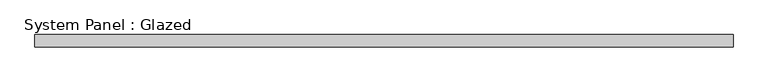
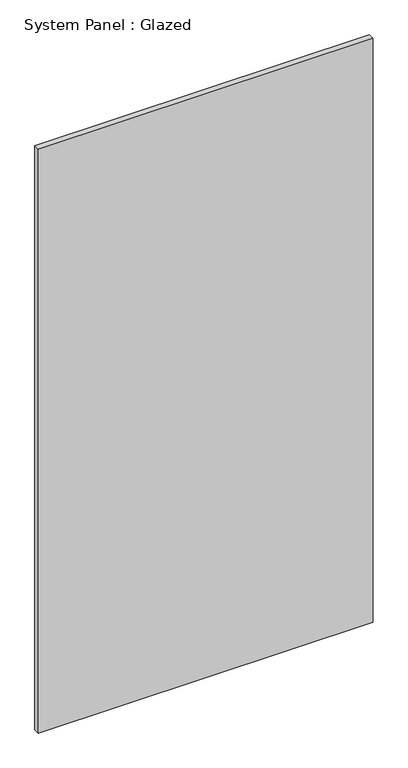
"""IFC4 building model written with IfcOpenShell, lengths in millimetres: plate geometry, System Panel : Glazed."""

import ifcopenshell
import ifcopenshell.guid

model = None  # the IFC model being written
_history = None  # IfcOwnerHistory: only IFC2X3 demands one
_inside = {}  # id of a spatial element -> (the spatial element, [elements in it])
_under = {}  # id of a project, library or spatial element -> (it, [spatial elements below it])
_declared = {}  # id of a project -> (the project, [libraries it declares])
_typed = {}  # id of a type object -> (the type object, [elements of that type])
_made_of = {}  # id of a material, layer set ... -> (it, [elements and type objects made of it])


def new_model(schema):
    """Start an empty IFC model of exactly this schema.

    Asked for "IFC4X3", IfcOpenShell would pick the latest addendum, in which some entities
    have other attributes; the version numbers below select the first issue.
    IFC2X3 requires an IfcOwnerHistory on every rooted entity: one is made here for all.
    """
    global model, _history
    if schema == "IFC4X3":
        model = ifcopenshell.file(schema_version=(4, 3, 0, 0))
    else:
        model = ifcopenshell.file(schema=schema)
    _inside.clear()
    _under.clear()
    _declared.clear()
    _typed.clear()
    _made_of.clear()
    _history = None
    if model.schema == "IFC2X3":
        org = make("IfcOrganization", Name="unknown")
        user = make(
            "IfcPersonAndOrganization",
            ThePerson=make("IfcPerson", FamilyName="unknown"),
            TheOrganization=org,
        )
        app = make(
            "IfcApplication",
            ApplicationDeveloper=org,
            Version="unknown",
            ApplicationFullName="unknown",
            ApplicationIdentifier="unknown",
        )
        _history = make(
            "IfcOwnerHistory",
            OwningUser=user,
            OwningApplication=app,
            ChangeAction="ADDED",
            CreationDate=0,
        )
    return model


def make(cls, **values):
    """One entity of the class cls with the attributes given. An attribute that is None is left unset."""
    return model.create_entity(
        cls, **{name: value for name, value in values.items() if value is not None}
    )


def rooted(cls, **values):
    """An entity with a GlobalId (a new one), such as an element, a storey or a relation."""
    return make(cls, GlobalId=ifcopenshell.guid.new(), OwnerHistory=_history, **values)


def si_unit(unit_type, name, prefix=None):
    """IfcSIUnit, for example si_unit("LENGTHUNIT", "METRE", prefix="MILLI")."""
    return make("IfcSIUnit", UnitType=unit_type, Prefix=prefix, Name=name)


def assignment(units):
    """IfcUnitAssignment: the units of a project."""
    return None if units is None else make("IfcUnitAssignment", Units=units)


def point(xyz):
    """IfcCartesianPoint."""
    return None if xyz is None else make("IfcCartesianPoint", Coordinates=xyz)


def direction(xyz):
    """IfcDirection."""
    return None if xyz is None else make("IfcDirection", DirectionRatios=xyz)


def frame(location, z_axis=None, x_axis=None):
    """IfcAxis2Placement3D, a coordinate frame: its origin and axes. An axis left out is left unset."""
    return make(
        "IfcAxis2Placement3D",
        Location=point(location),
        Axis=direction(z_axis),
        RefDirection=direction(x_axis),
    )


def origin():
    """The frame at (0, 0, 0) with its axes left unset."""
    return frame((0.0, 0.0, 0.0))


def origin_with_axes():
    """The frame at (0, 0, 0) with the z axis (0, 0, 1) and the x axis (1, 0, 0) written out."""
    return frame((0.0, 0.0, 0.0), z_axis=(0.0, 0.0, 1.0), x_axis=(1.0, 0.0, 0.0))


def place(relative_to, where):
    """IfcLocalPlacement: puts the frame where relative to a parent placement (None: the world)."""
    return make(
        "IfcLocalPlacement", PlacementRelTo=relative_to, RelativePlacement=where
    )


def context(
    kind, dimensions, precision=None, world=None, true_north=None, identifier=None
):
    """IfcGeometricRepresentationContext, for example the 3D "Model" context."""
    return make(
        "IfcGeometricRepresentationContext",
        ContextIdentifier=identifier,
        ContextType=kind,
        CoordinateSpaceDimension=dimensions,
        Precision=precision,
        WorldCoordinateSystem=world,
        TrueNorth=true_north,
    )


def project(units=None, contexts=None):
    """IfcProject with its units and contexts."""
    return rooted(
        "IfcProject",
        Name="project",
        RepresentationContexts=contexts,
        UnitsInContext=assignment(units),
    )


def spatial(cls, under=None, at=None, **own):
    """A site, building, storey or space (cls), placed at a placement, below another one or the project."""
    s = rooted(cls, ObjectPlacement=at, **own)
    if under is not None:
        _under.setdefault(under.id(), (under, []))[1].append(s)
    return s


def polyline(points):
    """IfcPolyline through the points."""
    return make("IfcPolyline", Points=[point(p) for p in points])


def outline(outer, holes=None, kind="AREA"):
    """IfcArbitraryClosedProfileDef: a profile drawn as a closed curve; with holes, ...WithVoids."""
    if holes is None:
        return make("IfcArbitraryClosedProfileDef", ProfileType=kind, OuterCurve=outer)
    return make(
        "IfcArbitraryProfileDefWithVoids",
        ProfileType=kind,
        OuterCurve=outer,
        InnerCurves=holes,
    )


def extrude(swept, where, along, depth):
    """IfcExtrudedAreaSolid: the profile swept, set in the frame where, extruded along a direction by depth."""
    return make(
        "IfcExtrudedAreaSolid",
        SweptArea=swept,
        Position=where,
        ExtrudedDirection=direction(along),
        Depth=depth,
    )


def shape(context_of_items, identifier, shape_type, items):
    """IfcShapeRepresentation: the items that make up one representation, for example the "Body"."""
    return make(
        "IfcShapeRepresentation",
        ContextOfItems=context_of_items,
        RepresentationIdentifier=identifier,
        RepresentationType=shape_type,
        Items=items,
    )


def source(mapping_origin, context_of_items, identifier, shape_type, items):
    """IfcRepresentationMap: a shape defined once, which mapped items show again and again."""
    return make(
        "IfcRepresentationMap",
        MappingOrigin=mapping_origin,
        MappedRepresentation=shape(context_of_items, identifier, shape_type, items),
    )


def transform(
    local_origin,
    x_axis=None,
    y_axis=None,
    z_axis=None,
    scale=None,
    scale2=None,
    scale3=None,
    uniform=True,
):
    """IfcCartesianTransformationOperator3D, or its non-uniform kind. x_axis, y_axis, z_axis: its Axis1, 2, 3."""
    if uniform:
        return make(
            "IfcCartesianTransformationOperator3D",
            Axis1=direction(x_axis),
            Axis2=direction(y_axis),
            LocalOrigin=point(local_origin),
            Scale=scale,
            Axis3=direction(z_axis),
        )
    return make(
        "IfcCartesianTransformationOperator3DnonUniform",
        Axis1=direction(x_axis),
        Axis2=direction(y_axis),
        LocalOrigin=point(local_origin),
        Scale=scale,
        Axis3=direction(z_axis),
        Scale2=scale2,
        Scale3=scale3,
    )


def mapped(mapping_source, mapping_target):
    """IfcMappedItem: shows the shape of a source again, moved by a transform."""
    return make(
        "IfcMappedItem", MappingSource=mapping_source, MappingTarget=mapping_target
    )


def made_of(thing, what):
    """Note that an element or type object is made of a material, layer set ...; save() writes the relation."""
    if what is not None:
        _made_of.setdefault(what.id(), (what, []))[1].append(thing)
    return thing


def element(
    cls,
    number,
    at=None,
    inside=None,
    cuts=None,
    type_object=None,
    material=None,
    context=None,
    identifier="Body",
    shape_type=None,
    held_by="IfcProductDefinitionShape",
    body=None,
    shapes=None,
    **own,
):
    """One element of the class cls, such as IfcWall. Its Tag is "e" and its number.

    at: its placement. inside: the storey or other place that contains it. cuts: it is an
    opening in that element (IfcRelVoidsElement). A single representation is given by context,
    identifier, shape_type and body (its items); several are given by shapes. held_by: the class
    of the entity that holds the representations. save() writes the other relations.
    """
    e = rooted(cls, Tag="e%d" % number, ObjectPlacement=at, **own)
    if body is not None:
        shapes = [shape(context, identifier, shape_type, body)]
    if shapes is not None:
        e.Representation = make(held_by, Representations=shapes)
    if inside is not None:
        _inside.setdefault(inside.id(), (inside, []))[1].append(e)
    if cuts is not None:
        rooted(
            "IfcRelVoidsElement", RelatingBuildingElement=cuts, RelatedOpeningElement=e
        )
    if type_object is not None:
        _typed.setdefault(type_object.id(), (type_object, []))[1].append(e)
    return made_of(e, material)


def aggregate(whole, parts):
    """IfcRelAggregates: a whole, such as a stair, and the parts it consists of."""
    return rooted("IfcRelAggregates", RelatingObject=whole, RelatedObjects=parts)


def save(model, path):
    """Write the relations noted so far, then the file.

    IfcRelAggregates (storeys below a building ...), IfcRelContainedInSpatialStructure (elements
    in a storey), IfcRelDefinesByType, IfcRelAssociatesMaterial and IfcRelDeclares: one each for
    every whole, place, type object, material and project.
    """
    for whole, parts in _under.values():
        aggregate(whole, parts)
    for where, things in _inside.values():
        rooted(
            "IfcRelContainedInSpatialStructure",
            RelatedElements=things,
            RelatingStructure=where,
        )
    for kind, things in _typed.values():
        rooted("IfcRelDefinesByType", RelatedObjects=things, RelatingType=kind)
    for what, things in _made_of.values():
        rooted("IfcRelAssociatesMaterial", RelatedObjects=things, RelatingMaterial=what)
    for by, libraries in _declared.values():
        rooted("IfcRelDeclares", RelatingContext=by, RelatedDefinitions=libraries)
    model.write(path)


def system_panel_glazed_ef639d2b(model_context):
    return source(origin(), model_context, "Body", "SweptSolid", [
        extrude(outline(polyline([(712.5000001, 24.5), (-712.5000001, 24.5), (-712.5000001, 49.5), (712.5000001, 49.5), (712.5000001, 24.5)])), origin_with_axes(), (0.0, 0.0, 1.0), 2625.0),
    ])


if __name__ == "__main__":
    model = new_model("IFC4")
    model_context = context("Model", 3, world=origin())
    ifc_project = project(units=[si_unit("LENGTHUNIT", "METRE", prefix="MILLI")], contexts=[model_context])
    site = spatial("IfcSite", under=ifc_project)
    building = spatial("IfcBuilding", under=site)
    placement = place(None, origin())
    system_panel_glazed_shape = system_panel_glazed_ef639d2b(model_context)
    element("IfcPlate", 1, ObjectType="System Panel : Glazed", at=placement, inside=building, context=model_context, shape_type="MappedRepresentation", body=[
        mapped(system_panel_glazed_shape, transform((0.0, 0.0, 0.0), x_axis=(1.0, 0.0, 0.0), y_axis=(0.0, 1.0, 0.0), z_axis=(0.0, 0.0, 1.0))),
    ])
    save(model, "model.ifc")

# Revit data of these elements
# Type "System Panel : Glazed"
#   Keynote = "H11"
#   Construction Type Id = "GSP4R"
#   Analytic Construction = "1/8 in Pilkington single glazing"
#   Visual Light Transmittance = 0.9
#   Solar Heat Gain Coefficient = 0.86
#   Heat Transfer Coefficient (U) = 6.7069 W/(m²·K)
# Element 1 (IfcPlate, "System Panel : Glazed")
#   Materials on its faces: "Glass"
# Materials
#   "Glass": class "Glass", colour RGB 0 128 192, transparency 0.9, Description = "Soda Lime Glass", Cost = 0
